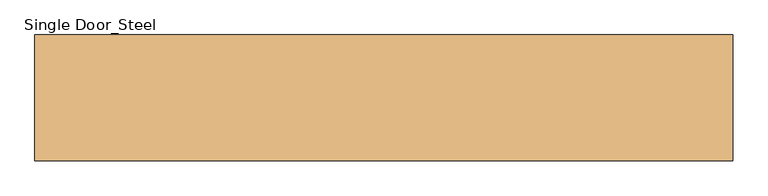
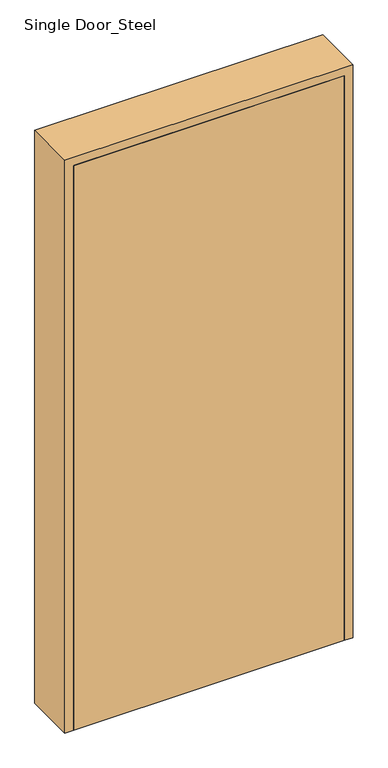
"""IFC4 building model written with IfcOpenShell, lengths in millimetres: door geometry, Single Door_Steel : H_DR_AR_B12_Single Door_Steel_W1000xH2100_0Hr."""

from ifc_helpers import new_model, si_unit, origin, origin_with_axes, place, context, project, spatial, polyline, outline, extrude, faceted_brep, source, transform, mapped, element, save


def single_door_steel_bbaeab1f(model_context):
    return source(origin(), model_context, "Body", "SolidModel", [
        extrude(outline(polyline([(470.0, -90.0), (-470.0, -90.0), (-470.0, -55.0), (470.0, -55.0), (470.0, -90.0)])), origin_with_axes(), (0.0, 0.0, 1.0), 2070.0),
        faceted_brep([(470.0, -90.0, 0.0), (470.0, -55.0, 0.0), (450.0, -55.0, 0.0), (450.0, 55.0, 0.0), (470.0, 55.0, 0.0), (470.0, 90.0, 0.0), (500.0, 90.0, 0.0), (500.0, -90.0, 0.0), (500.0, -90.0, 2100.0), (-500.0, -90.0, 2100.0), (-500.0, -90.0, 0.0), (-470.0, -90.0, 0.0), (-470.0, -90.0, 2070.0), (470.0, -90.0, 2070.0), (500.0, 90.0, 2100.0), (470.0, 90.0, 2070.0), (-470.0, 90.0, 2070.0), (-470.0, 90.0, 0.0), (-500.0, 90.0, 0.0), (-500.0, 90.0, 2100.0), (470.0, 55.0, 2070.0), (450.0, 55.0, 2050.0), (-450.0, 55.0, 2050.0), (-450.0, 55.0, 0.0), (-470.0, 55.0, 0.0), (-470.0, 55.0, 2070.0), (450.0, -55.0, 2050.0), (470.0, -55.0, 2070.0), (-470.0, -55.0, 2070.0), (-470.0, -55.0, 0.0), (-450.0, -55.0, 0.0), (-450.0, -55.0, 2050.0)], [[[0, 1, 2, 3, 4, 5, 6, 7]], [[7, 8, 9, 10, 11, 12, 13, 0]], [[6, 14, 8, 7]], [[5, 15, 16, 17, 18, 19, 14, 6]], [[4, 20, 15, 5]], [[3, 21, 22, 23, 24, 25, 20, 4]], [[2, 26, 21, 3]], [[1, 27, 28, 29, 30, 31, 26, 2]], [[0, 13, 27, 1]], [[12, 11, 29, 28]], [[11, 10, 18, 17, 24, 23, 30, 29]], [[19, 18, 10, 9]], [[25, 24, 17, 16]], [[31, 30, 23, 22]], [[14, 19, 9, 8]], [[20, 25, 16, 15]], [[26, 31, 22, 21]], [[13, 12, 28, 27]]]),
    ])


if __name__ == "__main__":
    model = new_model("IFC4")
    model_context = context("Model", 3, world=origin())
    ifc_project = project(units=[si_unit("LENGTHUNIT", "METRE", prefix="MILLI")], contexts=[model_context])
    site = spatial("IfcSite", under=ifc_project)
    building = spatial("IfcBuilding", under=site)
    placement = place(None, origin())
    single_door_steel_shape = single_door_steel_bbaeab1f(model_context)
    element("IfcDoor", 1, ObjectType="Single Door_Steel : H_DR_AR_B12_Single Door_Steel_W1000xH2100_0Hr", at=placement, inside=building, context=model_context, shape_type="MappedRepresentation", body=[
        mapped(single_door_steel_shape, transform((0.0, 0.0, 0.0), x_axis=(1.0, 0.0, 0.0), y_axis=(0.0, 1.0, 0.0), z_axis=(0.0, 0.0, 1.0))),
    ])
    save(model, "model.ifc")

# Revit data of these elements
# Type "Single Door_Steel : H_DR_AR_B12_Single Door_Steel_W1000xH2100_0Hr"
#   Type Mark = "SD1"
#   Analytic Construction = "<None>"
#   프레임 투영 외부. = 25 mm
#   프레임 투영 내부. = 25 mm
#   프레임 폭 = 75 mm
#   Height = 2100 mm
#   Width = 1000 mm
#   Define Thermal Properties by = 1
#   문 패널 = none
#   문 프레임 = none
#   Function = (empty or 0)
#   Wall Closure = (empty or 0)
